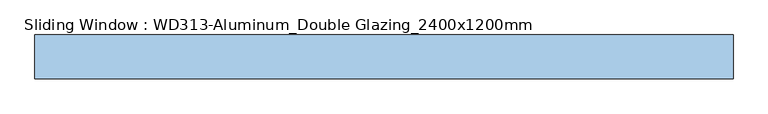
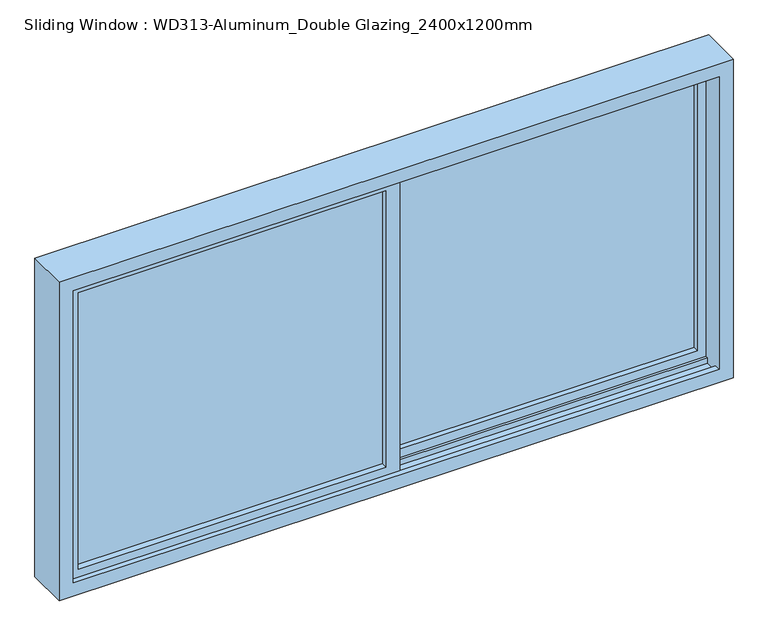
"""IFC4 building model written with IfcOpenShell, lengths in millimetres: window geometry, Sliding Window : WD313-Aluminum_Double Glazing_2400x1200mm."""

import ifcopenshell
import ifcopenshell.guid

model = None  # the IFC model being written
_history = None  # IfcOwnerHistory: only IFC2X3 demands one
_inside = {}  # id of a spatial element -> (the spatial element, [elements in it])
_under = {}  # id of a project, library or spatial element -> (it, [spatial elements below it])
_declared = {}  # id of a project -> (the project, [libraries it declares])
_typed = {}  # id of a type object -> (the type object, [elements of that type])
_made_of = {}  # id of a material, layer set ... -> (it, [elements and type objects made of it])


def new_model(schema):
    """Start an empty IFC model of exactly this schema.

    Asked for "IFC4X3", IfcOpenShell would pick the latest addendum, in which some entities
    have other attributes; the version numbers below select the first issue.
    IFC2X3 requires an IfcOwnerHistory on every rooted entity: one is made here for all.
    """
    global model, _history
    if schema == "IFC4X3":
        model = ifcopenshell.file(schema_version=(4, 3, 0, 0))
    else:
        model = ifcopenshell.file(schema=schema)
    _inside.clear()
    _under.clear()
    _declared.clear()
    _typed.clear()
    _made_of.clear()
    _history = None
    if model.schema == "IFC2X3":
        org = make("IfcOrganization", Name="unknown")
        user = make(
            "IfcPersonAndOrganization",
            ThePerson=make("IfcPerson", FamilyName="unknown"),
            TheOrganization=org,
        )
        app = make(
            "IfcApplication",
            ApplicationDeveloper=org,
            Version="unknown",
            ApplicationFullName="unknown",
            ApplicationIdentifier="unknown",
        )
        _history = make(
            "IfcOwnerHistory",
            OwningUser=user,
            OwningApplication=app,
            ChangeAction="ADDED",
            CreationDate=0,
        )
    return model


def make(cls, **values):
    """One entity of the class cls with the attributes given. An attribute that is None is left unset."""
    return model.create_entity(
        cls, **{name: value for name, value in values.items() if value is not None}
    )


def rooted(cls, **values):
    """An entity with a GlobalId (a new one), such as an element, a storey or a relation."""
    return make(cls, GlobalId=ifcopenshell.guid.new(), OwnerHistory=_history, **values)


def si_unit(unit_type, name, prefix=None):
    """IfcSIUnit, for example si_unit("LENGTHUNIT", "METRE", prefix="MILLI")."""
    return make("IfcSIUnit", UnitType=unit_type, Prefix=prefix, Name=name)


def assignment(units):
    """IfcUnitAssignment: the units of a project."""
    return None if units is None else make("IfcUnitAssignment", Units=units)


def point(xyz):
    """IfcCartesianPoint."""
    return None if xyz is None else make("IfcCartesianPoint", Coordinates=xyz)


def direction(xyz):
    """IfcDirection."""
    return None if xyz is None else make("IfcDirection", DirectionRatios=xyz)


def frame(location, z_axis=None, x_axis=None):
    """IfcAxis2Placement3D, a coordinate frame: its origin and axes. An axis left out is left unset."""
    return make(
        "IfcAxis2Placement3D",
        Location=point(location),
        Axis=direction(z_axis),
        RefDirection=direction(x_axis),
    )


def origin():
    """The frame at (0, 0, 0) with its axes left unset."""
    return frame((0.0, 0.0, 0.0))


def place(relative_to, where):
    """IfcLocalPlacement: puts the frame where relative to a parent placement (None: the world)."""
    return make(
        "IfcLocalPlacement", PlacementRelTo=relative_to, RelativePlacement=where
    )


def context(
    kind, dimensions, precision=None, world=None, true_north=None, identifier=None
):
    """IfcGeometricRepresentationContext, for example the 3D "Model" context."""
    return make(
        "IfcGeometricRepresentationContext",
        ContextIdentifier=identifier,
        ContextType=kind,
        CoordinateSpaceDimension=dimensions,
        Precision=precision,
        WorldCoordinateSystem=world,
        TrueNorth=true_north,
    )


def project(units=None, contexts=None):
    """IfcProject with its units and contexts."""
    return rooted(
        "IfcProject",
        Name="project",
        RepresentationContexts=contexts,
        UnitsInContext=assignment(units),
    )


def spatial(cls, under=None, at=None, **own):
    """A site, building, storey or space (cls), placed at a placement, below another one or the project."""
    s = rooted(cls, ObjectPlacement=at, **own)
    if under is not None:
        _under.setdefault(under.id(), (under, []))[1].append(s)
    return s


def polyline(points):
    """IfcPolyline through the points."""
    return make("IfcPolyline", Points=[point(p) for p in points])


def outline(outer, holes=None, kind="AREA"):
    """IfcArbitraryClosedProfileDef: a profile drawn as a closed curve; with holes, ...WithVoids."""
    if holes is None:
        return make("IfcArbitraryClosedProfileDef", ProfileType=kind, OuterCurve=outer)
    return make(
        "IfcArbitraryProfileDefWithVoids",
        ProfileType=kind,
        OuterCurve=outer,
        InnerCurves=holes,
    )


def extrude(swept, where, along, depth):
    """IfcExtrudedAreaSolid: the profile swept, set in the frame where, extruded along a direction by depth."""
    return make(
        "IfcExtrudedAreaSolid",
        SweptArea=swept,
        Position=where,
        ExtrudedDirection=direction(along),
        Depth=depth,
    )


def faces_of(points, faces, orient=None, outer=None):
    """IfcFace entities. A face is a list of loops; a loop is a list of indices into points, from 0.

    orient and outer hold one flag for each loop. By default every Orientation is true, the
    first loop of a face is its IfcFaceOuterBound and the others are IfcFaceBound.
    """
    made = []
    for i, loops in enumerate(faces):
        bounds = []
        for j, loop in enumerate(loops):
            is_outer = j == 0 if outer is None else outer[i][j]
            bounds.append(
                make(
                    "IfcFaceOuterBound" if is_outer else "IfcFaceBound",
                    Bound=make("IfcPolyLoop", Polygon=[points[k] for k in loop]),
                    Orientation=True if orient is None else orient[i][j],
                )
            )
        made.append(make("IfcFace", Bounds=bounds))
    return made


def faceted_brep(points, faces, orient=None, outer=None, voids=None):
    """IfcFacetedBrep: a solid bounded by flat faces; with voids (closed shells), ...WithVoids."""
    shared = [point(p) for p in points]
    hull = make("IfcClosedShell", CfsFaces=faces_of(shared, faces, orient, outer))
    if voids is None:
        return make("IfcFacetedBrep", Outer=hull)
    return make(
        "IfcFacetedBrepWithVoids",
        Outer=hull,
        Voids=[
            make(cls, CfsFaces=faces_of(shared, fs, o, b)) for cls, fs, o, b in voids
        ],
    )


def shape(context_of_items, identifier, shape_type, items):
    """IfcShapeRepresentation: the items that make up one representation, for example the "Body"."""
    return make(
        "IfcShapeRepresentation",
        ContextOfItems=context_of_items,
        RepresentationIdentifier=identifier,
        RepresentationType=shape_type,
        Items=items,
    )


def source(mapping_origin, context_of_items, identifier, shape_type, items):
    """IfcRepresentationMap: a shape defined once, which mapped items show again and again."""
    return make(
        "IfcRepresentationMap",
        MappingOrigin=mapping_origin,
        MappedRepresentation=shape(context_of_items, identifier, shape_type, items),
    )


def transform(
    local_origin,
    x_axis=None,
    y_axis=None,
    z_axis=None,
    scale=None,
    scale2=None,
    scale3=None,
    uniform=True,
):
    """IfcCartesianTransformationOperator3D, or its non-uniform kind. x_axis, y_axis, z_axis: its Axis1, 2, 3."""
    if uniform:
        return make(
            "IfcCartesianTransformationOperator3D",
            Axis1=direction(x_axis),
            Axis2=direction(y_axis),
            LocalOrigin=point(local_origin),
            Scale=scale,
            Axis3=direction(z_axis),
        )
    return make(
        "IfcCartesianTransformationOperator3DnonUniform",
        Axis1=direction(x_axis),
        Axis2=direction(y_axis),
        LocalOrigin=point(local_origin),
        Scale=scale,
        Axis3=direction(z_axis),
        Scale2=scale2,
        Scale3=scale3,
    )


def mapped(mapping_source, mapping_target):
    """IfcMappedItem: shows the shape of a source again, moved by a transform."""
    return make(
        "IfcMappedItem", MappingSource=mapping_source, MappingTarget=mapping_target
    )


def made_of(thing, what):
    """Note that an element or type object is made of a material, layer set ...; save() writes the relation."""
    if what is not None:
        _made_of.setdefault(what.id(), (what, []))[1].append(thing)
    return thing


def element(
    cls,
    number,
    at=None,
    inside=None,
    cuts=None,
    type_object=None,
    material=None,
    context=None,
    identifier="Body",
    shape_type=None,
    held_by="IfcProductDefinitionShape",
    body=None,
    shapes=None,
    **own,
):
    """One element of the class cls, such as IfcWall. Its Tag is "e" and its number.

    at: its placement. inside: the storey or other place that contains it. cuts: it is an
    opening in that element (IfcRelVoidsElement). A single representation is given by context,
    identifier, shape_type and body (its items); several are given by shapes. held_by: the class
    of the entity that holds the representations. save() writes the other relations.
    """
    e = rooted(cls, Tag="e%d" % number, ObjectPlacement=at, **own)
    if body is not None:
        shapes = [shape(context, identifier, shape_type, body)]
    if shapes is not None:
        e.Representation = make(held_by, Representations=shapes)
    if inside is not None:
        _inside.setdefault(inside.id(), (inside, []))[1].append(e)
    if cuts is not None:
        rooted(
            "IfcRelVoidsElement", RelatingBuildingElement=cuts, RelatedOpeningElement=e
        )
    if type_object is not None:
        _typed.setdefault(type_object.id(), (type_object, []))[1].append(e)
    return made_of(e, material)


def aggregate(whole, parts):
    """IfcRelAggregates: a whole, such as a stair, and the parts it consists of."""
    return rooted("IfcRelAggregates", RelatingObject=whole, RelatedObjects=parts)


def save(model, path):
    """Write the relations noted so far, then the file.

    IfcRelAggregates (storeys below a building ...), IfcRelContainedInSpatialStructure (elements
    in a storey), IfcRelDefinesByType, IfcRelAssociatesMaterial and IfcRelDeclares: one each for
    every whole, place, type object, material and project.
    """
    for whole, parts in _under.values():
        aggregate(whole, parts)
    for where, things in _inside.values():
        rooted(
            "IfcRelContainedInSpatialStructure",
            RelatedElements=things,
            RelatingStructure=where,
        )
    for kind, things in _typed.values():
        rooted("IfcRelDefinesByType", RelatedObjects=things, RelatingType=kind)
    for what, things in _made_of.values():
        rooted("IfcRelAssociatesMaterial", RelatedObjects=things, RelatingMaterial=what)
    for by, libraries in _declared.values():
        rooted("IfcRelDeclares", RelatingContext=by, RelatedDefinitions=libraries)
    model.write(path)


def sliding_window_wd313_aluminum_double_glazing_2400x1200mm_47b363be(model_context):
    return source(origin(), model_context, "Body", "SolidModel", [
        extrude(outline(polyline([(1120.0, 27.5), (25.0, 27.5), (25.0, 32.5), (1120.0, 32.5), (1120.0, 27.5)])), frame((0.0, 0.0, 680.0), z_axis=(0.0, 0.0, 1.0), x_axis=(1.0, 0.0, 0.0)), (0.0, 0.0, 1.0), 1040.0),
        extrude(outline(polyline([(-25.0, -32.5), (-1120.0, -32.5), (-1120.0, -27.5), (-25.0, -27.5), (-25.0, -32.5)])), frame((0.0, 0.0, 680.0), z_axis=(0.0, 0.0, 1.0), x_axis=(1.0, 0.0, 0.0)), (0.0, 0.0, 1.0), 1040.0),
        extrude(outline(polyline([(630.0, -1170.0), (630.0, 25.0), (1770.0, 25.0), (1770.0, -1170.0), (630.0, -1170.0)]), holes=[polyline([(1720.0, -1120.0), (1720.0, -25.0), (680.0, -25.0), (680.0, -1120.0), (1720.0, -1120.0)])]), frame((0.0, -55.0, 0.0), z_axis=(0.0, 1.0, 0.0), x_axis=(0.0, 0.0, 1.0)), (0.0, 0.0, 1.0), 47.5),
        extrude(outline(polyline([(630.0, -25.0), (630.0, 1170.0), (1770.0, 1170.0), (1770.0, -25.0), (630.0, -25.0)]), holes=[polyline([(1720.0, 25.0), (1720.0, 1120.0), (680.0, 1120.0), (680.0, 25.0), (1720.0, 25.0)])]), frame((0.0, 7.5, 0.0), z_axis=(0.0, 1.0, 0.0), x_axis=(0.0, 0.0, 1.0)), (0.0, 0.0, 1.0), 45.0),
        faceted_brep([(-1200.0, 75.0, 1800.0), (-1200.0, 75.0, 600.0), (-1200.0, -75.0, 600.0), (-1200.0, -75.0, 1800.0), (1200.0, 75.0, 1800.0), (1200.0, 75.0, 600.0), (1150.0, 75.0, 650.0), (1150.0, 75.0, 1750.0), (-1150.0, 75.0, 1750.0), (-1150.0, 75.0, 650.0), (1200.0, -75.0, 600.0), (1200.0, -75.0, 1800.0), (-1150.0, -75.0, 1750.0), (1150.0, -75.0, 1750.0), (1150.0, -75.0, 650.0), (-1150.0, -75.0, 650.0), (1150.0, 55.0, 650.0), (1150.0, 55.0, 1750.0), (-1150.0, 55.0, 1750.0), (-1150.0, 55.0, 1770.0), (-1150.0, 5.0, 1770.0), (-1150.0, 5.0, 1750.0), (-1150.0, -5.0, 1750.0), (-1150.0, -5.0, 650.0), (-1150.0, 5.0, 650.0), (-1150.0, 5.0, 630.0), (-1150.0, 55.0, 630.0), (-1150.0, 55.0, 650.0), (1150.0, -5.0, 650.0), (1150.0, 5.0, 650.0), (1150.0, -5.0, 630.0), (1150.0, -55.0, 630.0), (1150.0, -55.0, 650.0), (1150.0, -55.0, 1750.0), (1150.0, -55.0, 1770.0), (1150.0, -5.0, 1770.0), (1150.0, -5.0, 1750.0), (1150.0, 5.0, 1750.0), (1170.0, 5.0, 1770.0), (1170.0, 5.0, 630.0), (-1170.0, -5.0, 1770.0), (-1170.0, -5.0, 630.0), (1170.0, 55.0, 1770.0), (1170.0, 55.0, 630.0), (-1170.0, -55.0, 630.0), (-1150.0, -55.0, 1750.0), (-1150.0, -55.0, 650.0), (-1170.0, -55.0, 1770.0)], [[[0, 1, 2, 3]], [[4, 5, 1, 0], [6, 7, 8, 9]], [[1, 5, 10, 2]], [[10, 11, 3, 2], [12, 13, 14, 15]], [[7, 6, 16, 17]], [[9, 8, 18, 19, 20, 21, 22, 23, 24, 25, 26, 27]], [[16, 6, 9, 27]], [[5, 4, 11, 10]], [[28, 29, 24, 23]], [[28, 30, 31, 32, 14, 13, 33, 34, 35, 36, 37, 29]], [[29, 37, 21, 20, 38, 39, 25, 24]], [[40, 41, 30, 28, 23, 22, 36, 35]], [[39, 38, 42, 43]], [[39, 43, 26, 25]], [[43, 42, 19, 18, 17, 16, 27, 26]], [[41, 44, 31, 30]], [[45, 46, 32, 31, 44, 47, 34, 33]], [[46, 15, 14, 32]], [[12, 15, 46, 45]], [[47, 44, 41, 40]], [[3, 11, 4, 0]], [[37, 36, 22, 21]], [[42, 38, 20, 19]], [[7, 17, 18, 8]], [[12, 45, 33, 13]], [[47, 40, 35, 34]]]),
    ])


if __name__ == "__main__":
    model = new_model("IFC4")
    model_context = context("Model", 3, world=origin())
    ifc_project = project(units=[si_unit("LENGTHUNIT", "METRE", prefix="MILLI")], contexts=[model_context])
    site = spatial("IfcSite", under=ifc_project)
    building = spatial("IfcBuilding", under=site)
    placement = place(None, origin())
    sliding_window_wd313_aluminum_double_glazing_2400x1200mm_shape = sliding_window_wd313_aluminum_double_glazing_2400x1200mm_47b363be(model_context)
    element("IfcWindow", 1, ObjectType="Sliding Window : WD313-Aluminum_Double Glazing_2400x1200mm", at=placement, inside=building, context=model_context, shape_type="MappedRepresentation", body=[
        mapped(sliding_window_wd313_aluminum_double_glazing_2400x1200mm_shape, transform((0.0, 0.0, 0.0), x_axis=(1.0, 0.0, 0.0), y_axis=(0.0, 1.0, 0.0), z_axis=(0.0, 0.0, 1.0))),
    ])
    save(model, "model.ifc")

# Revit data of these elements
# Type "Sliding Window : WD313-Aluminum_Double Glazing_2400x1200mm"
#   Type Mark = "PW"
#   Analytic Construction = "<None>"
#   창 두께 = 150 mm
#   Visual Light Transmittance = 0.9
#   Thermal Resistance (R) = 0.271106 (m²·K)/W
#   Solar Heat Gain Coefficient = 0.78
#   Height = 1200 mm
#   Heat Transfer Coefficient (U) = 3.6886 W/(m²·K)
#   기본 씰 높이 = 600 mm
#   Width = 2400 mm
#   Define Thermal Properties by = 1
#   창 패널 = AW1 창 패널
#   창 프레임 = A04AQ127-00002_Aluminum Window_None FP
#   Description = (empty or 0)
#   Construction Type Id = ""
#   Wall Closure = (empty or 0)
# Element 1 (IfcWindow, "Sliding Window : WD313-Aluminum_Double Glazing_2400x1200mm")
#   Materials on its faces: "A04AQ127-00002_Aluminum Window_None FP", "AW1 창 패널"
# Materials
#   "AW1 창 패널": class "유리", colour RGB 0 0 255, transparency 0.75
#   "A04AQ127-00002_Aluminum Window_None FP": class "금속", colour RGB 247 247 247, transparency 0, W00) Work Master Code = "A04AQ127-00002", W01) Work Master_Lv1 = "Finishing Work", W02) Work Master_Lv2 = "Door & Window Work", W03) Work Master_Spec.1 = "Aluminum Window", W04) Work Master_Spec.2 = "Fire Protective Rating: N/A", W05) Work Master_Spec.3 = "w/ Hardware & Accessories", Cost = 0
